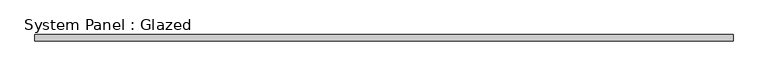
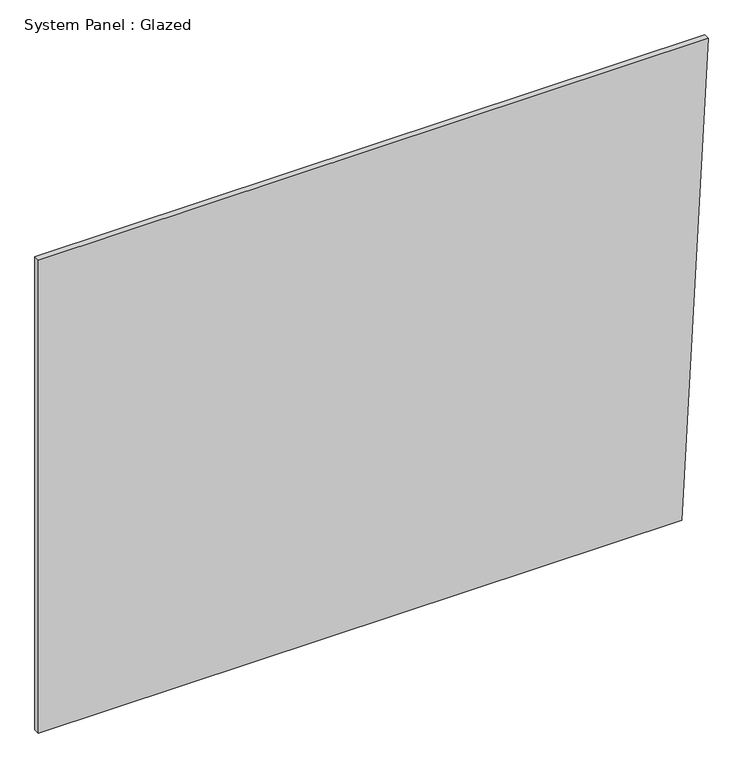
"""IFC4 building model written with IfcOpenShell, lengths in millimetres: plate geometry, System Panel : Glazed."""

import ifcopenshell
import ifcopenshell.guid

model = None  # the IFC model being written
_history = None  # IfcOwnerHistory: only IFC2X3 demands one
_inside = {}  # id of a spatial element -> (the spatial element, [elements in it])
_under = {}  # id of a project, library or spatial element -> (it, [spatial elements below it])
_declared = {}  # id of a project -> (the project, [libraries it declares])
_typed = {}  # id of a type object -> (the type object, [elements of that type])
_made_of = {}  # id of a material, layer set ... -> (it, [elements and type objects made of it])


def new_model(schema):
    """Start an empty IFC model of exactly this schema.

    Asked for "IFC4X3", IfcOpenShell would pick the latest addendum, in which some entities
    have other attributes; the version numbers below select the first issue.
    IFC2X3 requires an IfcOwnerHistory on every rooted entity: one is made here for all.
    """
    global model, _history
    if schema == "IFC4X3":
        model = ifcopenshell.file(schema_version=(4, 3, 0, 0))
    else:
        model = ifcopenshell.file(schema=schema)
    _inside.clear()
    _under.clear()
    _declared.clear()
    _typed.clear()
    _made_of.clear()
    _history = None
    if model.schema == "IFC2X3":
        org = make("IfcOrganization", Name="unknown")
        user = make(
            "IfcPersonAndOrganization",
            ThePerson=make("IfcPerson", FamilyName="unknown"),
            TheOrganization=org,
        )
        app = make(
            "IfcApplication",
            ApplicationDeveloper=org,
            Version="unknown",
            ApplicationFullName="unknown",
            ApplicationIdentifier="unknown",
        )
        _history = make(
            "IfcOwnerHistory",
            OwningUser=user,
            OwningApplication=app,
            ChangeAction="ADDED",
            CreationDate=0,
        )
    return model


def make(cls, **values):
    """One entity of the class cls with the attributes given. An attribute that is None is left unset."""
    return model.create_entity(
        cls, **{name: value for name, value in values.items() if value is not None}
    )


def rooted(cls, **values):
    """An entity with a GlobalId (a new one), such as an element, a storey or a relation."""
    return make(cls, GlobalId=ifcopenshell.guid.new(), OwnerHistory=_history, **values)


def si_unit(unit_type, name, prefix=None):
    """IfcSIUnit, for example si_unit("LENGTHUNIT", "METRE", prefix="MILLI")."""
    return make("IfcSIUnit", UnitType=unit_type, Prefix=prefix, Name=name)


def assignment(units):
    """IfcUnitAssignment: the units of a project."""
    return None if units is None else make("IfcUnitAssignment", Units=units)


def point(xyz):
    """IfcCartesianPoint."""
    return None if xyz is None else make("IfcCartesianPoint", Coordinates=xyz)


def direction(xyz):
    """IfcDirection."""
    return None if xyz is None else make("IfcDirection", DirectionRatios=xyz)


def frame(location, z_axis=None, x_axis=None):
    """IfcAxis2Placement3D, a coordinate frame: its origin and axes. An axis left out is left unset."""
    return make(
        "IfcAxis2Placement3D",
        Location=point(location),
        Axis=direction(z_axis),
        RefDirection=direction(x_axis),
    )


def origin():
    """The frame at (0, 0, 0) with its axes left unset."""
    return frame((0.0, 0.0, 0.0))


def place(relative_to, where):
    """IfcLocalPlacement: puts the frame where relative to a parent placement (None: the world)."""
    return make(
        "IfcLocalPlacement", PlacementRelTo=relative_to, RelativePlacement=where
    )


def context(
    kind, dimensions, precision=None, world=None, true_north=None, identifier=None
):
    """IfcGeometricRepresentationContext, for example the 3D "Model" context."""
    return make(
        "IfcGeometricRepresentationContext",
        ContextIdentifier=identifier,
        ContextType=kind,
        CoordinateSpaceDimension=dimensions,
        Precision=precision,
        WorldCoordinateSystem=world,
        TrueNorth=true_north,
    )


def project(units=None, contexts=None):
    """IfcProject with its units and contexts."""
    return rooted(
        "IfcProject",
        Name="project",
        RepresentationContexts=contexts,
        UnitsInContext=assignment(units),
    )


def spatial(cls, under=None, at=None, **own):
    """A site, building, storey or space (cls), placed at a placement, below another one or the project."""
    s = rooted(cls, ObjectPlacement=at, **own)
    if under is not None:
        _under.setdefault(under.id(), (under, []))[1].append(s)
    return s


def polyline(points):
    """IfcPolyline through the points."""
    return make("IfcPolyline", Points=[point(p) for p in points])


def outline(outer, holes=None, kind="AREA"):
    """IfcArbitraryClosedProfileDef: a profile drawn as a closed curve; with holes, ...WithVoids."""
    if holes is None:
        return make("IfcArbitraryClosedProfileDef", ProfileType=kind, OuterCurve=outer)
    return make(
        "IfcArbitraryProfileDefWithVoids",
        ProfileType=kind,
        OuterCurve=outer,
        InnerCurves=holes,
    )


def extrude(swept, where, along, depth):
    """IfcExtrudedAreaSolid: the profile swept, set in the frame where, extruded along a direction by depth."""
    return make(
        "IfcExtrudedAreaSolid",
        SweptArea=swept,
        Position=where,
        ExtrudedDirection=direction(along),
        Depth=depth,
    )


def shape(context_of_items, identifier, shape_type, items):
    """IfcShapeRepresentation: the items that make up one representation, for example the "Body"."""
    return make(
        "IfcShapeRepresentation",
        ContextOfItems=context_of_items,
        RepresentationIdentifier=identifier,
        RepresentationType=shape_type,
        Items=items,
    )


def source(mapping_origin, context_of_items, identifier, shape_type, items):
    """IfcRepresentationMap: a shape defined once, which mapped items show again and again."""
    return make(
        "IfcRepresentationMap",
        MappingOrigin=mapping_origin,
        MappedRepresentation=shape(context_of_items, identifier, shape_type, items),
    )


def transform(
    local_origin,
    x_axis=None,
    y_axis=None,
    z_axis=None,
    scale=None,
    scale2=None,
    scale3=None,
    uniform=True,
):
    """IfcCartesianTransformationOperator3D, or its non-uniform kind. x_axis, y_axis, z_axis: its Axis1, 2, 3."""
    if uniform:
        return make(
            "IfcCartesianTransformationOperator3D",
            Axis1=direction(x_axis),
            Axis2=direction(y_axis),
            LocalOrigin=point(local_origin),
            Scale=scale,
            Axis3=direction(z_axis),
        )
    return make(
        "IfcCartesianTransformationOperator3DnonUniform",
        Axis1=direction(x_axis),
        Axis2=direction(y_axis),
        LocalOrigin=point(local_origin),
        Scale=scale,
        Axis3=direction(z_axis),
        Scale2=scale2,
        Scale3=scale3,
    )


def mapped(mapping_source, mapping_target):
    """IfcMappedItem: shows the shape of a source again, moved by a transform."""
    return make(
        "IfcMappedItem", MappingSource=mapping_source, MappingTarget=mapping_target
    )


def made_of(thing, what):
    """Note that an element or type object is made of a material, layer set ...; save() writes the relation."""
    if what is not None:
        _made_of.setdefault(what.id(), (what, []))[1].append(thing)
    return thing


def element(
    cls,
    number,
    at=None,
    inside=None,
    cuts=None,
    type_object=None,
    material=None,
    context=None,
    identifier="Body",
    shape_type=None,
    held_by="IfcProductDefinitionShape",
    body=None,
    shapes=None,
    **own,
):
    """One element of the class cls, such as IfcWall. Its Tag is "e" and its number.

    at: its placement. inside: the storey or other place that contains it. cuts: it is an
    opening in that element (IfcRelVoidsElement). A single representation is given by context,
    identifier, shape_type and body (its items); several are given by shapes. held_by: the class
    of the entity that holds the representations. save() writes the other relations.
    """
    e = rooted(cls, Tag="e%d" % number, ObjectPlacement=at, **own)
    if body is not None:
        shapes = [shape(context, identifier, shape_type, body)]
    if shapes is not None:
        e.Representation = make(held_by, Representations=shapes)
    if inside is not None:
        _inside.setdefault(inside.id(), (inside, []))[1].append(e)
    if cuts is not None:
        rooted(
            "IfcRelVoidsElement", RelatingBuildingElement=cuts, RelatedOpeningElement=e
        )
    if type_object is not None:
        _typed.setdefault(type_object.id(), (type_object, []))[1].append(e)
    return made_of(e, material)


def aggregate(whole, parts):
    """IfcRelAggregates: a whole, such as a stair, and the parts it consists of."""
    return rooted("IfcRelAggregates", RelatingObject=whole, RelatedObjects=parts)


def save(model, path):
    """Write the relations noted so far, then the file.

    IfcRelAggregates (storeys below a building ...), IfcRelContainedInSpatialStructure (elements
    in a storey), IfcRelDefinesByType, IfcRelAssociatesMaterial and IfcRelDeclares: one each for
    every whole, place, type object, material and project.
    """
    for whole, parts in _under.values():
        aggregate(whole, parts)
    for where, things in _inside.values():
        rooted(
            "IfcRelContainedInSpatialStructure",
            RelatedElements=things,
            RelatingStructure=where,
        )
    for kind, things in _typed.values():
        rooted("IfcRelDefinesByType", RelatedObjects=things, RelatingType=kind)
    for what, things in _made_of.values():
        rooted("IfcRelAssociatesMaterial", RelatedObjects=things, RelatingMaterial=what)
    for by, libraries in _declared.values():
        rooted("IfcRelDeclares", RelatingContext=by, RelatedDefinitions=libraries)
    model.write(path)


def system_panel_glazed_3b2a3880(model_context):
    return source(origin(), model_context, "Body", "SweptSolid", [
        extrude(outline(polyline([(0.0, -1396.3622347), (0.0, 1287.2219516), (2085.3785982, 1396.3622347), (2085.3785982, -1396.3622347), (0.0, -1396.3622347)])), frame((0.0, -44.45, 0.0), z_axis=(0.0, 1.0, 0.0), x_axis=(0.0, 0.0, 1.0)), (0.0, 0.0, 1.0), 25.4),
    ])


if __name__ == "__main__":
    model = new_model("IFC4")
    model_context = context("Model", 3, world=origin())
    ifc_project = project(units=[si_unit("LENGTHUNIT", "METRE", prefix="MILLI")], contexts=[model_context])
    site = spatial("IfcSite", under=ifc_project)
    building = spatial("IfcBuilding", under=site)
    placement = place(None, origin())
    system_panel_glazed_shape = system_panel_glazed_3b2a3880(model_context)
    element("IfcPlate", 1, ObjectType="System Panel : Glazed", at=placement, inside=building, context=model_context, shape_type="MappedRepresentation", body=[
        mapped(system_panel_glazed_shape, transform((0.0, 0.0, 0.0), x_axis=(1.0, 0.0, 0.0), y_axis=(0.0, 1.0, 0.0), z_axis=(0.0, 0.0, 1.0))),
    ])
    save(model, "model.ifc")

# Revit data of these elements
# Type "System Panel : Glazed"
#   Construction Type Id = "GSP4R"
#   Analytic Construction = "1/8 in Pilkington single glazing"
#   Visual Light Transmittance = 0.9
#   Solar Heat Gain Coefficient = 0.86
#   Heat Transfer Coefficient (U) = 1.18115 BTU/(h·ft²·°F)
#   Define Thermal Properties by = 1
# Element 1 (IfcPlate, "System Panel : Glazed")
#   Materials on its faces: "Glass"
# Materials
#   "Glass": class "Glass", colour RGB 0 128 192, transparency 0.75, Description = "Soda Lime Glass", Cost = 0
